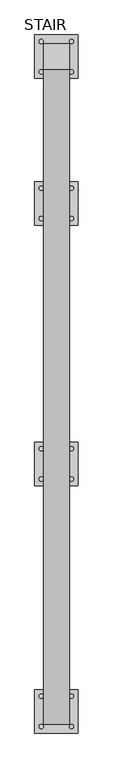
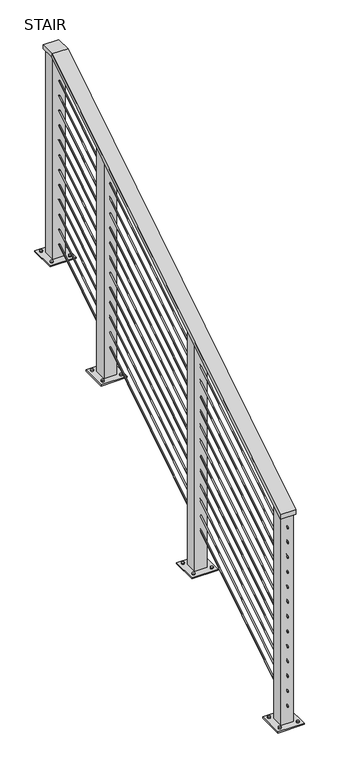
"""IFC4 building model written with IfcOpenShell, lengths in millimetres: railing geometry, STAIR."""

from ifc_helpers import new_model, si_unit, point, frame, frame_2d, origin, place, context, project, spatial, polyline, circle_curve, ellipse_curve, trimmed, segment, composite_curve, outline, extrude, faceted_brep, source, transform, mapped, element, save
from ifc_brep_helpers import plane_surface, cylinder_surface, advanced_brep


def stair_dfb8d1b2(model_context):
    return source(origin(), model_context, "Body", "SolidModel", [
        faceted_brep([(27131.1620052, 3906.3043237, 2667.5780048), (27054.9620052, 3906.3043237, 2667.5780048), (27054.9620052, 3906.3043237, 2645.0989839), (27131.1620052, 3906.3043237, 2645.0989839), (27131.1620052, 5821.2673274, 3867.15), (27054.9620052, 5821.2673274, 3867.15), (27054.9620052, 5826.7413199, 3848.1), (27131.1620052, 5826.7413199, 3848.1), (27131.1620052, 5897.4594438, 3867.15), (27131.1620052, 5897.4594438, 3848.1), (27054.9620052, 5897.4594438, 3848.1), (27054.9620052, 5897.4594438, 3867.15)], [[[0, 1, 2, 3]], [[1, 0, 4, 5]], [[2, 1, 5, 6]], [[3, 2, 6, 7]], [[0, 3, 7, 4]], [[8, 9, 10, 11]], [[5, 4, 8, 11]], [[6, 5, 11, 10]], [[7, 6, 10, 9]], [[4, 7, 9, 8]]]),
        advanced_brep(
        [(27090.6807552, 3906.3043237, 2586.8536167), (27095.4432552, 3906.3043237, 2586.8536167), (27090.6807552, 5824.6885727, 3788.56875), (27095.4432552, 5824.6885727, 3788.56875), (27090.6807552, 5897.4594438, 3788.56875), (27095.4432552, 5897.4594438, 3788.56875)],
        [
            (0, 1, ellipse_curve(frame((27093.0620052, 3906.3043237, 2586.8536167), z_axis=(0.0, -1.0, 0.0), x_axis=(0.0, 0.0, -1.0)), 2.8098776, 2.38125)),
            (1, 0, ellipse_curve(frame((27093.0620052, 3906.3043237, 2586.8536167), z_axis=(0.0, -1.0, 0.0), x_axis=(0.0, 0.0, -1.0)), 2.8098776, 2.38125)),
            (0, 2),
            (2, 3, ellipse_curve(frame((27093.0620052, 5824.6885727, 3788.56875), z_axis=(0.0, -0.9611079128273461, -0.27617309771348614), x_axis=(0.0, 0.27617309771348714, -0.9611079128273459)), 2.4776094, 2.38125)),
            (3, 1),
            (3, 2, ellipse_curve(frame((27093.0620052, 5824.6885727, 3788.56875), z_axis=(0.0, -0.9611079128273461, -0.27617309771348614), x_axis=(0.0, 0.27617309771348714, -0.9611079128273459)), 2.4776094, 2.38125)),
            (4, 5, circle_curve(frame((27093.0620052, 5897.4594438, 3788.56875), z_axis=(0.0, 1.0, 0.0), x_axis=(1.0, 0.0, 0.0)), 2.38125)),
            (5, 4, circle_curve(frame((27093.0620052, 5897.4594438, 3788.56875), z_axis=(0.0, 1.0, 0.0), x_axis=(1.0, 0.0, 0.0)), 2.38125)),
            (2, 4),
            (5, 3),
        ],
        [
            plane_surface(frame((27093.0620052, 3906.3043237, 2589.6634943), z_axis=(0.0, -1.0, 0.0), x_axis=(0.0, 0.0, 1.0))),
            cylinder_surface(frame((27093.0620052, 3907.5684443, 2587.6454877), z_axis=(0.0, -0.8474568401986745, -0.5308642990449426), x_axis=(1.0, 0.0, 0.0)), 2.38125),
            plane_surface(frame((27093.0620052, 5897.4594438, 3790.95), z_axis=(0.0, 1.0, 0.0), x_axis=(0.0, 0.0, 1.0))),
            cylinder_surface(frame((27093.0620052, 5824.0043237, 3788.56875), z_axis=(0.0, -1.0, 0.0), x_axis=(1.0, 0.0, 0.0)), 2.38125),
        ],
        [
            (0, [[1, 2]]),
            (1, [[-1, 3, 4, 5]]),
            (1, [[-2, -5, 6, -3]]),
            (2, [[7, 8]]),
            (3, [[-4, 9, -8, 10]]),
            (3, [[-6, -10, -7, -9]]),
        ],
    ),
        advanced_brep(
        [(27090.6807552, 3906.3043237, 2510.6536167), (27095.4432552, 3906.3043237, 2510.6536167), (27090.6807552, 5824.6885727, 3712.36875), (27095.4432552, 5824.6885727, 3712.36875), (27090.6807552, 5897.4594438, 3712.36875), (27095.4432552, 5897.4594438, 3712.36875)],
        [
            (0, 1, ellipse_curve(frame((27093.0620052, 3906.3043237, 2510.6536167), z_axis=(0.0, -1.0, 0.0), x_axis=(0.0, 0.0, -1.0)), 2.8098776, 2.38125)),
            (1, 0, ellipse_curve(frame((27093.0620052, 3906.3043237, 2510.6536167), z_axis=(0.0, -1.0, 0.0), x_axis=(0.0, 0.0, -1.0)), 2.8098776, 2.38125)),
            (0, 2),
            (2, 3, ellipse_curve(frame((27093.0620052, 5824.6885727, 3712.36875), z_axis=(0.0, -0.9611079128273461, -0.27617309771348614), x_axis=(0.0, 0.27617309771348714, -0.9611079128273459)), 2.4776094, 2.38125)),
            (3, 1),
            (3, 2, ellipse_curve(frame((27093.0620052, 5824.6885727, 3712.36875), z_axis=(0.0, -0.9611079128273461, -0.27617309771348614), x_axis=(0.0, 0.27617309771348714, -0.9611079128273459)), 2.4776094, 2.38125)),
            (4, 5, circle_curve(frame((27093.0620052, 5897.4594438, 3712.36875), z_axis=(0.0, 1.0, 0.0), x_axis=(1.0, 0.0, 0.0)), 2.38125)),
            (5, 4, circle_curve(frame((27093.0620052, 5897.4594438, 3712.36875), z_axis=(0.0, 1.0, 0.0), x_axis=(1.0, 0.0, 0.0)), 2.38125)),
            (2, 4),
            (5, 3),
        ],
        [
            plane_surface(frame((27093.0620052, 3906.3043237, 2513.4634943), z_axis=(0.0, -1.0, 0.0), x_axis=(0.0, 0.0, 1.0))),
            cylinder_surface(frame((27093.0620052, 3907.5684443, 2511.4454877), z_axis=(0.0, -0.8474568401986745, -0.5308642990449426), x_axis=(1.0, 0.0, 0.0)), 2.38125),
            plane_surface(frame((27093.0620052, 5897.4594438, 3714.75), z_axis=(0.0, 1.0, 0.0), x_axis=(0.0, 0.0, 1.0))),
            cylinder_surface(frame((27093.0620052, 5824.0043237, 3712.36875), z_axis=(0.0, -1.0, 0.0), x_axis=(1.0, 0.0, 0.0)), 2.38125),
        ],
        [
            (0, [[1, 2]]),
            (1, [[-1, 3, 4, 5]]),
            (1, [[-2, -5, 6, -3]]),
            (2, [[7, 8]]),
            (3, [[-4, 9, -8, 10]]),
            (3, [[-6, -10, -7, -9]]),
        ],
    ),
        advanced_brep(
        [(27090.6807552, 3906.3043237, 2434.4536167), (27095.4432552, 3906.3043237, 2434.4536167), (27090.6807552, 5824.6885727, 3636.16875), (27095.4432552, 5824.6885727, 3636.16875), (27090.6807552, 5897.4594438, 3636.16875), (27095.4432552, 5897.4594438, 3636.16875)],
        [
            (0, 1, ellipse_curve(frame((27093.0620052, 3906.3043237, 2434.4536167), z_axis=(0.0, -1.0, 0.0), x_axis=(0.0, 0.0, -1.0)), 2.8098776, 2.38125)),
            (1, 0, ellipse_curve(frame((27093.0620052, 3906.3043237, 2434.4536167), z_axis=(0.0, -1.0, 0.0), x_axis=(0.0, 0.0, -1.0)), 2.8098776, 2.38125)),
            (0, 2),
            (2, 3, ellipse_curve(frame((27093.0620052, 5824.6885727, 3636.16875), z_axis=(0.0, -0.9611079128273461, -0.27617309771348614), x_axis=(0.0, 0.27617309771348714, -0.9611079128273459)), 2.4776094, 2.38125)),
            (3, 1),
            (3, 2, ellipse_curve(frame((27093.0620052, 5824.6885727, 3636.16875), z_axis=(0.0, -0.9611079128273461, -0.27617309771348614), x_axis=(0.0, 0.27617309771348714, -0.9611079128273459)), 2.4776094, 2.38125)),
            (4, 5, circle_curve(frame((27093.0620052, 5897.4594438, 3636.16875), z_axis=(0.0, 1.0, 0.0), x_axis=(1.0, 0.0, 0.0)), 2.38125)),
            (5, 4, circle_curve(frame((27093.0620052, 5897.4594438, 3636.16875), z_axis=(0.0, 1.0, 0.0), x_axis=(1.0, 0.0, 0.0)), 2.38125)),
            (2, 4),
            (5, 3),
        ],
        [
            plane_surface(frame((27093.0620052, 3906.3043237, 2437.2634943), z_axis=(0.0, -1.0, 0.0), x_axis=(0.0, 0.0, 1.0))),
            cylinder_surface(frame((27093.0620052, 3907.5684443, 2435.2454877), z_axis=(0.0, -0.8474568401986745, -0.5308642990449426), x_axis=(1.0, 0.0, 0.0)), 2.38125),
            plane_surface(frame((27093.0620052, 5897.4594438, 3638.55), z_axis=(0.0, 1.0, 0.0), x_axis=(0.0, 0.0, 1.0))),
            cylinder_surface(frame((27093.0620052, 5824.0043237, 3636.16875), z_axis=(0.0, -1.0, 0.0), x_axis=(1.0, 0.0, 0.0)), 2.38125),
        ],
        [
            (0, [[1, 2]]),
            (1, [[-1, 3, 4, 5]]),
            (1, [[-2, -5, 6, -3]]),
            (2, [[7, 8]]),
            (3, [[-4, 9, -8, 10]]),
            (3, [[-6, -10, -7, -9]]),
        ],
    ),
        advanced_brep(
        [(27090.6807552, 3906.3043237, 2358.2536167), (27095.4432552, 3906.3043237, 2358.2536167), (27090.6807552, 5824.6885727, 3559.96875), (27095.4432552, 5824.6885727, 3559.96875), (27090.6807552, 5897.4594438, 3559.96875), (27095.4432552, 5897.4594438, 3559.96875)],
        [
            (0, 1, ellipse_curve(frame((27093.0620052, 3906.3043237, 2358.2536167), z_axis=(0.0, -1.0, 0.0), x_axis=(0.0, 0.0, -1.0)), 2.8098776, 2.38125)),
            (1, 0, ellipse_curve(frame((27093.0620052, 3906.3043237, 2358.2536167), z_axis=(0.0, -1.0, 0.0), x_axis=(0.0, 0.0, -1.0)), 2.8098776, 2.38125)),
            (0, 2),
            (2, 3, ellipse_curve(frame((27093.0620052, 5824.6885727, 3559.96875), z_axis=(0.0, -0.9611079128273461, -0.27617309771348614), x_axis=(0.0, 0.27617309771348714, -0.9611079128273459)), 2.4776094, 2.38125)),
            (3, 1),
            (3, 2, ellipse_curve(frame((27093.0620052, 5824.6885727, 3559.96875), z_axis=(0.0, -0.9611079128273461, -0.27617309771348614), x_axis=(0.0, 0.27617309771348714, -0.9611079128273459)), 2.4776094, 2.38125)),
            (4, 5, circle_curve(frame((27093.0620052, 5897.4594438, 3559.96875), z_axis=(0.0, 1.0, 0.0), x_axis=(1.0, 0.0, 0.0)), 2.38125)),
            (5, 4, circle_curve(frame((27093.0620052, 5897.4594438, 3559.96875), z_axis=(0.0, 1.0, 0.0), x_axis=(1.0, 0.0, 0.0)), 2.38125)),
            (2, 4),
            (5, 3),
        ],
        [
            plane_surface(frame((27093.0620052, 3906.3043237, 2361.0634943), z_axis=(0.0, -1.0, 0.0), x_axis=(0.0, 0.0, 1.0))),
            cylinder_surface(frame((27093.0620052, 3907.5684443, 2359.0454877), z_axis=(0.0, -0.8474568401986745, -0.5308642990449426), x_axis=(1.0, 0.0, 0.0)), 2.38125),
            plane_surface(frame((27093.0620052, 5897.4594438, 3562.35), z_axis=(0.0, 1.0, 0.0), x_axis=(0.0, 0.0, 1.0))),
            cylinder_surface(frame((27093.0620052, 5824.0043237, 3559.96875), z_axis=(0.0, -1.0, 0.0), x_axis=(1.0, 0.0, 0.0)), 2.38125),
        ],
        [
            (0, [[1, 2]]),
            (1, [[-1, 3, 4, 5]]),
            (1, [[-2, -5, 6, -3]]),
            (2, [[7, 8]]),
            (3, [[-4, 9, -8, 10]]),
            (3, [[-6, -10, -7, -9]]),
        ],
    ),
        advanced_brep(
        [(27090.6807552, 3906.3043237, 2282.0536167), (27095.4432552, 3906.3043237, 2282.0536167), (27090.6807552, 5824.6885727, 3483.76875), (27095.4432552, 5824.6885727, 3483.76875), (27090.6807552, 5897.4594438, 3483.76875), (27095.4432552, 5897.4594438, 3483.76875)],
        [
            (0, 1, ellipse_curve(frame((27093.0620052, 3906.3043237, 2282.0536167), z_axis=(0.0, -1.0, 0.0), x_axis=(0.0, 0.0, -1.0)), 2.8098776, 2.38125)),
            (1, 0, ellipse_curve(frame((27093.0620052, 3906.3043237, 2282.0536167), z_axis=(0.0, -1.0, 0.0), x_axis=(0.0, 0.0, -1.0)), 2.8098776, 2.38125)),
            (0, 2),
            (2, 3, ellipse_curve(frame((27093.0620052, 5824.6885727, 3483.76875), z_axis=(0.0, -0.9611079128273461, -0.27617309771348614), x_axis=(0.0, 0.27617309771348714, -0.9611079128273459)), 2.4776094, 2.38125)),
            (3, 1),
            (3, 2, ellipse_curve(frame((27093.0620052, 5824.6885727, 3483.76875), z_axis=(0.0, -0.9611079128273461, -0.27617309771348614), x_axis=(0.0, 0.27617309771348714, -0.9611079128273459)), 2.4776094, 2.38125)),
            (4, 5, circle_curve(frame((27093.0620052, 5897.4594438, 3483.76875), z_axis=(0.0, 1.0, 0.0), x_axis=(1.0, 0.0, 0.0)), 2.38125)),
            (5, 4, circle_curve(frame((27093.0620052, 5897.4594438, 3483.76875), z_axis=(0.0, 1.0, 0.0), x_axis=(1.0, 0.0, 0.0)), 2.38125)),
            (2, 4),
            (5, 3),
        ],
        [
            plane_surface(frame((27093.0620052, 3906.3043237, 2284.8634943), z_axis=(0.0, -1.0, 0.0), x_axis=(0.0, 0.0, 1.0))),
            cylinder_surface(frame((27093.0620052, 3907.5684443, 2282.8454877), z_axis=(0.0, -0.8474568401986745, -0.5308642990449426), x_axis=(1.0, 0.0, 0.0)), 2.38125),
            plane_surface(frame((27093.0620052, 5897.4594438, 3486.15), z_axis=(0.0, 1.0, 0.0), x_axis=(0.0, 0.0, 1.0))),
            cylinder_surface(frame((27093.0620052, 5824.0043237, 3483.76875), z_axis=(0.0, -1.0, 0.0), x_axis=(1.0, 0.0, 0.0)), 2.38125),
        ],
        [
            (0, [[1, 2]]),
            (1, [[-1, 3, 4, 5]]),
            (1, [[-2, -5, 6, -3]]),
            (2, [[7, 8]]),
            (3, [[-4, 9, -8, 10]]),
            (3, [[-6, -10, -7, -9]]),
        ],
    ),
        advanced_brep(
        [(27090.6807552, 3906.3043237, 2205.8536167), (27095.4432552, 3906.3043237, 2205.8536167), (27090.6807552, 5824.6885727, 3407.56875), (27095.4432552, 5824.6885727, 3407.56875), (27090.6807552, 5897.4594438, 3407.56875), (27095.4432552, 5897.4594438, 3407.56875)],
        [
            (0, 1, ellipse_curve(frame((27093.0620052, 3906.3043237, 2205.8536167), z_axis=(0.0, -1.0, 0.0), x_axis=(0.0, 0.0, -1.0)), 2.8098776, 2.38125)),
            (1, 0, ellipse_curve(frame((27093.0620052, 3906.3043237, 2205.8536167), z_axis=(0.0, -1.0, 0.0), x_axis=(0.0, 0.0, -1.0)), 2.8098776, 2.38125)),
            (0, 2),
            (2, 3, ellipse_curve(frame((27093.0620052, 5824.6885727, 3407.56875), z_axis=(0.0, -0.9611079128273461, -0.27617309771348614), x_axis=(0.0, 0.27617309771348714, -0.9611079128273459)), 2.4776094, 2.38125)),
            (3, 1),
            (3, 2, ellipse_curve(frame((27093.0620052, 5824.6885727, 3407.56875), z_axis=(0.0, -0.9611079128273461, -0.27617309771348614), x_axis=(0.0, 0.27617309771348714, -0.9611079128273459)), 2.4776094, 2.38125)),
            (4, 5, circle_curve(frame((27093.0620052, 5897.4594438, 3407.56875), z_axis=(0.0, 1.0, 0.0), x_axis=(1.0, 0.0, 0.0)), 2.38125)),
            (5, 4, circle_curve(frame((27093.0620052, 5897.4594438, 3407.56875), z_axis=(0.0, 1.0, 0.0), x_axis=(1.0, 0.0, 0.0)), 2.38125)),
            (2, 4),
            (5, 3),
        ],
        [
            plane_surface(frame((27093.0620052, 3906.3043237, 2208.6634943), z_axis=(0.0, -1.0, 0.0), x_axis=(0.0, 0.0, 1.0))),
            cylinder_surface(frame((27093.0620052, 3907.5684443, 2206.6454877), z_axis=(0.0, -0.8474568401986745, -0.5308642990449426), x_axis=(1.0, 0.0, 0.0)), 2.38125),
            plane_surface(frame((27093.0620052, 5897.4594438, 3409.95), z_axis=(0.0, 1.0, 0.0), x_axis=(0.0, 0.0, 1.0))),
            cylinder_surface(frame((27093.0620052, 5824.0043237, 3407.56875), z_axis=(0.0, -1.0, 0.0), x_axis=(1.0, 0.0, 0.0)), 2.38125),
        ],
        [
            (0, [[1, 2]]),
            (1, [[-1, 3, 4, 5]]),
            (1, [[-2, -5, 6, -3]]),
            (2, [[7, 8]]),
            (3, [[-4, 9, -8, 10]]),
            (3, [[-6, -10, -7, -9]]),
        ],
    ),
        advanced_brep(
        [(27090.6807552, 3906.3043237, 2129.6536167), (27095.4432552, 3906.3043237, 2129.6536167), (27090.6807552, 5824.6885727, 3331.36875), (27095.4432552, 5824.6885727, 3331.36875), (27090.6807552, 5897.4594438, 3331.36875), (27095.4432552, 5897.4594438, 3331.36875)],
        [
            (0, 1, ellipse_curve(frame((27093.0620052, 3906.3043237, 2129.6536167), z_axis=(0.0, -1.0, 0.0), x_axis=(0.0, 0.0, -1.0)), 2.8098776, 2.38125)),
            (1, 0, ellipse_curve(frame((27093.0620052, 3906.3043237, 2129.6536167), z_axis=(0.0, -1.0, 0.0), x_axis=(0.0, 0.0, -1.0)), 2.8098776, 2.38125)),
            (0, 2),
            (2, 3, ellipse_curve(frame((27093.0620052, 5824.6885727, 3331.36875), z_axis=(0.0, -0.9611079128273461, -0.27617309771348614), x_axis=(0.0, 0.27617309771348714, -0.9611079128273459)), 2.4776094, 2.38125)),
            (3, 1),
            (3, 2, ellipse_curve(frame((27093.0620052, 5824.6885727, 3331.36875), z_axis=(0.0, -0.9611079128273461, -0.27617309771348614), x_axis=(0.0, 0.27617309771348714, -0.9611079128273459)), 2.4776094, 2.38125)),
            (4, 5, circle_curve(frame((27093.0620052, 5897.4594438, 3331.36875), z_axis=(0.0, 1.0, 0.0), x_axis=(1.0, 0.0, 0.0)), 2.38125)),
            (5, 4, circle_curve(frame((27093.0620052, 5897.4594438, 3331.36875), z_axis=(0.0, 1.0, 0.0), x_axis=(1.0, 0.0, 0.0)), 2.38125)),
            (2, 4),
            (5, 3),
        ],
        [
            plane_surface(frame((27093.0620052, 3906.3043237, 2132.4634943), z_axis=(0.0, -1.0, 0.0), x_axis=(0.0, 0.0, 1.0))),
            cylinder_surface(frame((27093.0620052, 3907.5684443, 2130.4454877), z_axis=(0.0, -0.8474568401986745, -0.5308642990449426), x_axis=(1.0, 0.0, 0.0)), 2.38125),
            plane_surface(frame((27093.0620052, 5897.4594438, 3333.75), z_axis=(0.0, 1.0, 0.0), x_axis=(0.0, 0.0, 1.0))),
            cylinder_surface(frame((27093.0620052, 5824.0043237, 3331.36875), z_axis=(0.0, -1.0, 0.0), x_axis=(1.0, 0.0, 0.0)), 2.38125),
        ],
        [
            (0, [[1, 2]]),
            (1, [[-1, 3, 4, 5]]),
            (1, [[-2, -5, 6, -3]]),
            (2, [[7, 8]]),
            (3, [[-4, 9, -8, 10]]),
            (3, [[-6, -10, -7, -9]]),
        ],
    ),
        advanced_brep(
        [(27090.6807552, 3906.3043237, 2053.4536167), (27095.4432552, 3906.3043237, 2053.4536167), (27090.6807552, 5824.6885727, 3255.16875), (27095.4432552, 5824.6885727, 3255.16875), (27090.6807552, 5897.4594438, 3255.16875), (27095.4432552, 5897.4594438, 3255.16875)],
        [
            (0, 1, ellipse_curve(frame((27093.0620052, 3906.3043237, 2053.4536167), z_axis=(0.0, -1.0, 0.0), x_axis=(0.0, 0.0, -1.0)), 2.8098776, 2.38125)),
            (1, 0, ellipse_curve(frame((27093.0620052, 3906.3043237, 2053.4536167), z_axis=(0.0, -1.0, 0.0), x_axis=(0.0, 0.0, -1.0)), 2.8098776, 2.38125)),
            (0, 2),
            (2, 3, ellipse_curve(frame((27093.0620052, 5824.6885727, 3255.16875), z_axis=(0.0, -0.9611079128273461, -0.27617309771348614), x_axis=(0.0, 0.27617309771348714, -0.9611079128273459)), 2.4776094, 2.38125)),
            (3, 1),
            (3, 2, ellipse_curve(frame((27093.0620052, 5824.6885727, 3255.16875), z_axis=(0.0, -0.9611079128273461, -0.27617309771348614), x_axis=(0.0, 0.27617309771348714, -0.9611079128273459)), 2.4776094, 2.38125)),
            (4, 5, circle_curve(frame((27093.0620052, 5897.4594438, 3255.16875), z_axis=(0.0, 1.0, 0.0), x_axis=(1.0, 0.0, 0.0)), 2.38125)),
            (5, 4, circle_curve(frame((27093.0620052, 5897.4594438, 3255.16875), z_axis=(0.0, 1.0, 0.0), x_axis=(1.0, 0.0, 0.0)), 2.38125)),
            (2, 4),
            (5, 3),
        ],
        [
            plane_surface(frame((27093.0620052, 3906.3043237, 2056.2634943), z_axis=(0.0, -1.0, 0.0), x_axis=(0.0, 0.0, 1.0))),
            cylinder_surface(frame((27093.0620052, 3907.5684443, 2054.2454877), z_axis=(0.0, -0.8474568401986745, -0.5308642990449426), x_axis=(1.0, 0.0, 0.0)), 2.38125),
            plane_surface(frame((27093.0620052, 5897.4594438, 3257.55), z_axis=(0.0, 1.0, 0.0), x_axis=(0.0, 0.0, 1.0))),
            cylinder_surface(frame((27093.0620052, 5824.0043237, 3255.16875), z_axis=(0.0, -1.0, 0.0), x_axis=(1.0, 0.0, 0.0)), 2.38125),
        ],
        [
            (0, [[1, 2]]),
            (1, [[-1, 3, 4, 5]]),
            (1, [[-2, -5, 6, -3]]),
            (2, [[7, 8]]),
            (3, [[-4, 9, -8, 10]]),
            (3, [[-6, -10, -7, -9]]),
        ],
    ),
        advanced_brep(
        [(27090.6807552, 3906.3043237, 1977.2536167), (27095.4432552, 3906.3043237, 1977.2536167), (27090.6807552, 5824.6885727, 3178.96875), (27095.4432552, 5824.6885727, 3178.96875), (27090.6807552, 5897.4594438, 3178.96875), (27095.4432552, 5897.4594438, 3178.96875)],
        [
            (0, 1, ellipse_curve(frame((27093.0620052, 3906.3043237, 1977.2536167), z_axis=(0.0, -1.0, 0.0), x_axis=(0.0, 0.0, -1.0)), 2.8098776, 2.38125)),
            (1, 0, ellipse_curve(frame((27093.0620052, 3906.3043237, 1977.2536167), z_axis=(0.0, -1.0, 0.0), x_axis=(0.0, 0.0, -1.0)), 2.8098776, 2.38125)),
            (0, 2),
            (2, 3, ellipse_curve(frame((27093.0620052, 5824.6885727, 3178.96875), z_axis=(0.0, -0.9611079128273461, -0.27617309771348614), x_axis=(0.0, 0.27617309771348714, -0.9611079128273459)), 2.4776094, 2.38125)),
            (3, 1),
            (3, 2, ellipse_curve(frame((27093.0620052, 5824.6885727, 3178.96875), z_axis=(0.0, -0.9611079128273461, -0.27617309771348614), x_axis=(0.0, 0.27617309771348714, -0.9611079128273459)), 2.4776094, 2.38125)),
            (4, 5, circle_curve(frame((27093.0620052, 5897.4594438, 3178.96875), z_axis=(0.0, 1.0, 0.0), x_axis=(1.0, 0.0, 0.0)), 2.38125)),
            (5, 4, circle_curve(frame((27093.0620052, 5897.4594438, 3178.96875), z_axis=(0.0, 1.0, 0.0), x_axis=(1.0, 0.0, 0.0)), 2.38125)),
            (2, 4),
            (5, 3),
        ],
        [
            plane_surface(frame((27093.0620052, 3906.3043237, 1980.0634943), z_axis=(0.0, -1.0, 0.0), x_axis=(0.0, 0.0, 1.0))),
            cylinder_surface(frame((27093.0620052, 3907.5684443, 1978.0454877), z_axis=(0.0, -0.8474568401986745, -0.5308642990449426), x_axis=(1.0, 0.0, 0.0)), 2.38125),
            plane_surface(frame((27093.0620052, 5897.4594438, 3181.35), z_axis=(0.0, 1.0, 0.0), x_axis=(0.0, 0.0, 1.0))),
            cylinder_surface(frame((27093.0620052, 5824.0043237, 3178.96875), z_axis=(0.0, -1.0, 0.0), x_axis=(1.0, 0.0, 0.0)), 2.38125),
        ],
        [
            (0, [[1, 2]]),
            (1, [[-1, 3, 4, 5]]),
            (1, [[-2, -5, 6, -3]]),
            (2, [[7, 8]]),
            (3, [[-4, 9, -8, 10]]),
            (3, [[-6, -10, -7, -9]]),
        ],
    ),
        advanced_brep(
        [(27090.6807552, 3906.3043237, 1901.0536167), (27095.4432552, 3906.3043237, 1901.0536167), (27090.6807552, 5824.6885727, 3102.76875), (27095.4432552, 5824.6885727, 3102.76875), (27090.6807552, 5897.4594438, 3102.76875), (27095.4432552, 5897.4594438, 3102.76875)],
        [
            (0, 1, ellipse_curve(frame((27093.0620052, 3906.3043237, 1901.0536167), z_axis=(0.0, -1.0, 0.0), x_axis=(0.0, 0.0, -1.0)), 2.8098776, 2.38125)),
            (1, 0, ellipse_curve(frame((27093.0620052, 3906.3043237, 1901.0536167), z_axis=(0.0, -1.0, 0.0), x_axis=(0.0, 0.0, -1.0)), 2.8098776, 2.38125)),
            (0, 2),
            (2, 3, ellipse_curve(frame((27093.0620052, 5824.6885727, 3102.76875), z_axis=(0.0, -0.9611079128273461, -0.27617309771348614), x_axis=(0.0, 0.27617309771348714, -0.9611079128273459)), 2.4776094, 2.38125)),
            (3, 1),
            (3, 2, ellipse_curve(frame((27093.0620052, 5824.6885727, 3102.76875), z_axis=(0.0, -0.9611079128273461, -0.27617309771348614), x_axis=(0.0, 0.27617309771348714, -0.9611079128273459)), 2.4776094, 2.38125)),
            (4, 5, circle_curve(frame((27093.0620052, 5897.4594438, 3102.76875), z_axis=(0.0, 1.0, 0.0), x_axis=(1.0, 0.0, 0.0)), 2.38125)),
            (5, 4, circle_curve(frame((27093.0620052, 5897.4594438, 3102.76875), z_axis=(0.0, 1.0, 0.0), x_axis=(1.0, 0.0, 0.0)), 2.38125)),
            (2, 4),
            (5, 3),
        ],
        [
            plane_surface(frame((27093.0620052, 3906.3043237, 1903.8634943), z_axis=(0.0, -1.0, 0.0), x_axis=(0.0, 0.0, 1.0))),
            cylinder_surface(frame((27093.0620052, 3907.5684443, 1901.8454877), z_axis=(0.0, -0.8474568401986745, -0.5308642990449426), x_axis=(1.0, 0.0, 0.0)), 2.38125),
            plane_surface(frame((27093.0620052, 5897.4594438, 3105.15), z_axis=(0.0, 1.0, 0.0), x_axis=(0.0, 0.0, 1.0))),
            cylinder_surface(frame((27093.0620052, 5824.0043237, 3102.76875), z_axis=(0.0, -1.0, 0.0), x_axis=(1.0, 0.0, 0.0)), 2.38125),
        ],
        [
            (0, [[1, 2]]),
            (1, [[-1, 3, 4, 5]]),
            (1, [[-2, -5, 6, -3]]),
            (2, [[7, 8]]),
            (3, [[-4, 9, -8, 10]]),
            (3, [[-6, -10, -7, -9]]),
        ],
    ),
        advanced_brep(
        [(27090.6807552, 3906.3043237, 1824.8536167), (27095.4432552, 3906.3043237, 1824.8536167), (27090.6807552, 5824.6885727, 3026.56875), (27095.4432552, 5824.6885727, 3026.56875), (27090.6807552, 5897.4594438, 3026.56875), (27095.4432552, 5897.4594438, 3026.56875)],
        [
            (0, 1, ellipse_curve(frame((27093.0620052, 3906.3043237, 1824.8536167), z_axis=(0.0, -1.0, 0.0), x_axis=(0.0, 0.0, -1.0)), 2.8098776, 2.38125)),
            (1, 0, ellipse_curve(frame((27093.0620052, 3906.3043237, 1824.8536167), z_axis=(0.0, -1.0, 0.0), x_axis=(0.0, 0.0, -1.0)), 2.8098776, 2.38125)),
            (0, 2),
            (2, 3, ellipse_curve(frame((27093.0620052, 5824.6885727, 3026.56875), z_axis=(0.0, -0.9611079128273461, -0.27617309771348614), x_axis=(0.0, 0.27617309771348714, -0.9611079128273459)), 2.4776094, 2.38125)),
            (3, 1),
            (3, 2, ellipse_curve(frame((27093.0620052, 5824.6885727, 3026.56875), z_axis=(0.0, -0.9611079128273461, -0.27617309771348614), x_axis=(0.0, 0.27617309771348714, -0.9611079128273459)), 2.4776094, 2.38125)),
            (4, 5, circle_curve(frame((27093.0620052, 5897.4594438, 3026.56875), z_axis=(0.0, 1.0, 0.0), x_axis=(1.0, 0.0, 0.0)), 2.38125)),
            (5, 4, circle_curve(frame((27093.0620052, 5897.4594438, 3026.56875), z_axis=(0.0, 1.0, 0.0), x_axis=(1.0, 0.0, 0.0)), 2.38125)),
            (2, 4),
            (5, 3),
        ],
        [
            plane_surface(frame((27093.0620052, 3906.3043237, 1827.6634943), z_axis=(0.0, -1.0, 0.0), x_axis=(0.0, 0.0, 1.0))),
            cylinder_surface(frame((27093.0620052, 3907.5684443, 1825.6454877), z_axis=(0.0, -0.8474568401986745, -0.5308642990449426), x_axis=(1.0, 0.0, 0.0)), 2.38125),
            plane_surface(frame((27093.0620052, 5897.4594438, 3028.95), z_axis=(0.0, 1.0, 0.0), x_axis=(0.0, 0.0, 1.0))),
            cylinder_surface(frame((27093.0620052, 5824.0043237, 3026.56875), z_axis=(0.0, -1.0, 0.0), x_axis=(1.0, 0.0, 0.0)), 2.38125),
        ],
        [
            (0, [[1, 2]]),
            (1, [[-1, 3, 4, 5]]),
            (1, [[-2, -5, 6, -3]]),
            (2, [[7, 8]]),
            (3, [[-4, 9, -8, 10]]),
            (3, [[-6, -10, -7, -9]]),
        ],
    ),
        advanced_brep(
        [(27090.6807552, 3906.3043237, 1748.6536167), (27095.4432552, 3906.3043237, 1748.6536167), (27090.6807552, 5824.6885727, 2950.36875), (27095.4432552, 5824.6885727, 2950.36875), (27090.6807552, 5897.4594438, 2950.36875), (27095.4432552, 5897.4594438, 2950.36875)],
        [
            (0, 1, ellipse_curve(frame((27093.0620052, 3906.3043237, 1748.6536167), z_axis=(0.0, -1.0, 0.0), x_axis=(0.0, 0.0, -1.0)), 2.8098776, 2.38125)),
            (1, 0, ellipse_curve(frame((27093.0620052, 3906.3043237, 1748.6536167), z_axis=(0.0, -1.0, 0.0), x_axis=(0.0, 0.0, -1.0)), 2.8098776, 2.38125)),
            (0, 2),
            (2, 3, ellipse_curve(frame((27093.0620052, 5824.6885727, 2950.36875), z_axis=(0.0, -0.9611079128273461, -0.27617309771348614), x_axis=(0.0, 0.27617309771348714, -0.9611079128273459)), 2.4776094, 2.38125)),
            (3, 1),
            (3, 2, ellipse_curve(frame((27093.0620052, 5824.6885727, 2950.36875), z_axis=(0.0, -0.9611079128273461, -0.27617309771348614), x_axis=(0.0, 0.27617309771348714, -0.9611079128273459)), 2.4776094, 2.38125)),
            (4, 5, circle_curve(frame((27093.0620052, 5897.4594438, 2950.36875), z_axis=(0.0, 1.0, 0.0), x_axis=(1.0, 0.0, 0.0)), 2.38125)),
            (5, 4, circle_curve(frame((27093.0620052, 5897.4594438, 2950.36875), z_axis=(0.0, 1.0, 0.0), x_axis=(1.0, 0.0, 0.0)), 2.38125)),
            (2, 4),
            (5, 3),
        ],
        [
            plane_surface(frame((27093.0620052, 3906.3043237, 1751.4634943), z_axis=(0.0, -1.0, 0.0), x_axis=(0.0, 0.0, 1.0))),
            cylinder_surface(frame((27093.0620052, 3907.5684443, 1749.4454877), z_axis=(0.0, -0.8474568401986745, -0.5308642990449426), x_axis=(1.0, 0.0, 0.0)), 2.38125),
            plane_surface(frame((27093.0620052, 5897.4594438, 2952.75), z_axis=(0.0, 1.0, 0.0), x_axis=(0.0, 0.0, 1.0))),
            cylinder_surface(frame((27093.0620052, 5824.0043237, 2950.36875), z_axis=(0.0, -1.0, 0.0), x_axis=(1.0, 0.0, 0.0)), 2.38125),
        ],
        [
            (0, [[1, 2]]),
            (1, [[-1, 3, 4, 5]]),
            (1, [[-2, -5, 6, -3]]),
            (2, [[7, 8]]),
            (3, [[-4, 9, -8, 10]]),
            (3, [[-6, -10, -7, -9]]),
        ],
    ),
        advanced_brep(
        [(27090.6807552, 3906.3043237, 1672.4536167), (27095.4432552, 3906.3043237, 1672.4536167), (27090.6807552, 5824.6885727, 2874.16875), (27095.4432552, 5824.6885727, 2874.16875), (27090.6807552, 5897.4594438, 2874.16875), (27095.4432552, 5897.4594438, 2874.16875)],
        [
            (0, 1, ellipse_curve(frame((27093.0620052, 3906.3043237, 1672.4536167), z_axis=(0.0, -1.0, 0.0), x_axis=(0.0, 0.0, -1.0)), 2.8098776, 2.38125)),
            (1, 0, ellipse_curve(frame((27093.0620052, 3906.3043237, 1672.4536167), z_axis=(0.0, -1.0, 0.0), x_axis=(0.0, 0.0, -1.0)), 2.8098776, 2.38125)),
            (0, 2),
            (2, 3, ellipse_curve(frame((27093.0620052, 5824.6885727, 2874.16875), z_axis=(0.0, -0.9611079128273461, -0.27617309771348614), x_axis=(0.0, 0.27617309771348714, -0.9611079128273459)), 2.4776094, 2.38125)),
            (3, 1),
            (3, 2, ellipse_curve(frame((27093.0620052, 5824.6885727, 2874.16875), z_axis=(0.0, -0.9611079128273461, -0.27617309771348614), x_axis=(0.0, 0.27617309771348714, -0.9611079128273459)), 2.4776094, 2.38125)),
            (4, 5, circle_curve(frame((27093.0620052, 5897.4594438, 2874.16875), z_axis=(0.0, 1.0, 0.0), x_axis=(1.0, 0.0, 0.0)), 2.38125)),
            (5, 4, circle_curve(frame((27093.0620052, 5897.4594438, 2874.16875), z_axis=(0.0, 1.0, 0.0), x_axis=(1.0, 0.0, 0.0)), 2.38125)),
            (2, 4),
            (5, 3),
        ],
        [
            plane_surface(frame((27093.0620052, 3906.3043237, 1675.2634943), z_axis=(0.0, -1.0, 0.0), x_axis=(0.0, 0.0, 1.0))),
            cylinder_surface(frame((27093.0620052, 3907.5684443, 1673.2454877), z_axis=(0.0, -0.8474568401986745, -0.5308642990449426), x_axis=(1.0, 0.0, 0.0)), 2.38125),
            plane_surface(frame((27093.0620052, 5897.4594438, 2876.55), z_axis=(0.0, 1.0, 0.0), x_axis=(0.0, 0.0, 1.0))),
            cylinder_surface(frame((27093.0620052, 5824.0043237, 2874.16875), z_axis=(0.0, -1.0, 0.0), x_axis=(1.0, 0.0, 0.0)), 2.38125),
        ],
        [
            (0, [[1, 2]]),
            (1, [[-1, 3, 4, 5]]),
            (1, [[-2, -5, 6, -3]]),
            (2, [[7, 8]]),
            (3, [[-4, 9, -8, 10]]),
            (3, [[-6, -10, -7, -9]]),
        ],
    ),
        extrude(outline(composite_curve([segment(trimmed(circle_curve(frame_2d((27137.5120052, 5385.8543237)), 6.35), [point((27143.8620052, 5385.8543237))], [point((27131.1620052, 5385.8543237))], False, "CARTESIAN"), True, "CONTINUOUS"), segment(trimmed(circle_curve(frame_2d((27137.5120052, 5385.8543237)), 6.35), [point((27131.1620052, 5385.8543237))], [point((27143.8620052, 5385.8543237))], False, "CARTESIAN"), True, "CONTINUOUS")], self_intersect=False)), frame((0.0, 0.0, 2450.30625), z_axis=(0.0, 0.0, 1.0), x_axis=(1.0, 0.0, 0.0)), (0.0, 0.0, 1.0), 12.7),
        extrude(outline(composite_curve([segment(trimmed(circle_curve(frame_2d((27048.6120052, 5385.8543237)), 6.35), [point((27054.9620052, 5385.8543237))], [point((27042.2620052, 5385.8543237))], False, "CARTESIAN"), True, "CONTINUOUS"), segment(trimmed(circle_curve(frame_2d((27048.6120052, 5385.8543237)), 6.35), [point((27042.2620052, 5385.8543237))], [point((27054.9620052, 5385.8543237))], False, "CARTESIAN"), True, "CONTINUOUS")], self_intersect=False)), frame((0.0, 0.0, 2450.30625), z_axis=(0.0, 0.0, 1.0), x_axis=(1.0, 0.0, 0.0)), (0.0, 0.0, 1.0), 12.7),
        extrude(outline(composite_curve([segment(trimmed(circle_curve(frame_2d((27137.5120052, 5474.7543237)), 6.35), [point((27143.8620052, 5474.7543237))], [point((27131.1620052, 5474.7543237))], False, "CARTESIAN"), True, "CONTINUOUS"), segment(trimmed(circle_curve(frame_2d((27137.5120052, 5474.7543237)), 6.35), [point((27131.1620052, 5474.7543237))], [point((27143.8620052, 5474.7543237))], False, "CARTESIAN"), True, "CONTINUOUS")], self_intersect=False)), frame((0.0, 0.0, 2450.30625), z_axis=(0.0, 0.0, 1.0), x_axis=(1.0, 0.0, 0.0)), (0.0, 0.0, 1.0), 12.7),
        extrude(outline(composite_curve([segment(trimmed(circle_curve(frame_2d((27048.6120052, 5474.7543237)), 6.35), [point((27054.9620052, 5474.7543237))], [point((27042.2620052, 5474.7543237))], False, "CARTESIAN"), True, "CONTINUOUS"), segment(trimmed(circle_curve(frame_2d((27048.6120052, 5474.7543237)), 6.35), [point((27042.2620052, 5474.7543237))], [point((27054.9620052, 5474.7543237))], False, "CARTESIAN"), True, "CONTINUOUS")], self_intersect=False)), frame((0.0, 0.0, 2450.30625), z_axis=(0.0, 0.0, 1.0), x_axis=(1.0, 0.0, 0.0)), (0.0, 0.0, 1.0), 12.7),
        extrude(outline(polyline([(27029.5620052, 5366.8043237), (27029.5620052, 5493.8043237), (27156.5620052, 5493.8043237), (27156.5620052, 5366.8043237), (27029.5620052, 5366.8043237)])), frame((0.0, 0.0, 2450.30625), z_axis=(0.0, 0.0, 1.0), x_axis=(1.0, 0.0, 0.0)), (0.0, 0.0, 1.0), 6.35),
        extrude(outline(polyline([(27062.8995052, 5400.1418237), (27062.8995052, 5460.4668237), (27123.2245052, 5460.4668237), (27123.2245052, 5400.1418237), (27062.8995052, 5400.1418237)]), holes=[polyline([(27069.2495052, 5406.4918237), (27116.8745052, 5406.4918237), (27116.8745052, 5454.1168237), (27069.2495052, 5454.1168237), (27069.2495052, 5406.4918237)])]), frame((0.0, 0.0, 2450.30625), z_axis=(0.0, 0.0, 1.0), x_axis=(1.0, 0.0, 0.0)), (0.0, 0.0, 1.0), 1151.172017),
        extrude(outline(composite_curve([segment(trimmed(circle_curve(frame_2d((27137.5120052, 4623.8543237)), 6.35), [point((27143.8620052, 4623.8543237))], [point((27131.1620052, 4623.8543237))], False, "CARTESIAN"), True, "CONTINUOUS"), segment(trimmed(circle_curve(frame_2d((27137.5120052, 4623.8543237)), 6.35), [point((27131.1620052, 4623.8543237))], [point((27143.8620052, 4623.8543237))], False, "CARTESIAN"), True, "CONTINUOUS")], self_intersect=False)), frame((0.0, 0.0, 1925.240625), z_axis=(0.0, 0.0, 1.0), x_axis=(1.0, 0.0, 0.0)), (0.0, 0.0, 1.0), 12.7),
        extrude(outline(composite_curve([segment(trimmed(circle_curve(frame_2d((27048.6120052, 4623.8543237)), 6.35), [point((27054.9620052, 4623.8543237))], [point((27042.2620052, 4623.8543237))], False, "CARTESIAN"), True, "CONTINUOUS"), segment(trimmed(circle_curve(frame_2d((27048.6120052, 4623.8543237)), 6.35), [point((27042.2620052, 4623.8543237))], [point((27054.9620052, 4623.8543237))], False, "CARTESIAN"), True, "CONTINUOUS")], self_intersect=False)), frame((0.0, 0.0, 1925.240625), z_axis=(0.0, 0.0, 1.0), x_axis=(1.0, 0.0, 0.0)), (0.0, 0.0, 1.0), 12.7),
        extrude(outline(composite_curve([segment(trimmed(circle_curve(frame_2d((27137.5120052, 4712.7543237)), 6.35), [point((27143.8620052, 4712.7543237))], [point((27131.1620052, 4712.7543237))], False, "CARTESIAN"), True, "CONTINUOUS"), segment(trimmed(circle_curve(frame_2d((27137.5120052, 4712.7543237)), 6.35), [point((27131.1620052, 4712.7543237))], [point((27143.8620052, 4712.7543237))], False, "CARTESIAN"), True, "CONTINUOUS")], self_intersect=False)), frame((0.0, 0.0, 1925.240625), z_axis=(0.0, 0.0, 1.0), x_axis=(1.0, 0.0, 0.0)), (0.0, 0.0, 1.0), 12.7),
        extrude(outline(composite_curve([segment(trimmed(circle_curve(frame_2d((27048.6120052, 4712.7543237)), 6.35), [point((27054.9620052, 4712.7543237))], [point((27042.2620052, 4712.7543237))], False, "CARTESIAN"), True, "CONTINUOUS"), segment(trimmed(circle_curve(frame_2d((27048.6120052, 4712.7543237)), 6.35), [point((27042.2620052, 4712.7543237))], [point((27054.9620052, 4712.7543237))], False, "CARTESIAN"), True, "CONTINUOUS")], self_intersect=False)), frame((0.0, 0.0, 1925.240625), z_axis=(0.0, 0.0, 1.0), x_axis=(1.0, 0.0, 0.0)), (0.0, 0.0, 1.0), 12.7),
        extrude(outline(polyline([(27029.5620052, 4604.8043237), (27029.5620052, 4731.8043237), (27156.5620052, 4731.8043237), (27156.5620052, 4604.8043237), (27029.5620052, 4604.8043237)])), frame((0.0, 0.0, 1925.240625), z_axis=(0.0, 0.0, 1.0), x_axis=(1.0, 0.0, 0.0)), (0.0, 0.0, 1.0), 6.35),
        extrude(outline(polyline([(27062.8995052, 4638.1418237), (27062.8995052, 4698.4668237), (27123.2245052, 4698.4668237), (27123.2245052, 4638.1418237), (27062.8995052, 4638.1418237)]), holes=[polyline([(27069.2495052, 4644.4918237), (27116.8745052, 4644.4918237), (27116.8745052, 4692.1168237), (27069.2495052, 4692.1168237), (27069.2495052, 4644.4918237)])]), frame((0.0, 0.0, 1925.240625), z_axis=(0.0, 0.0, 1.0), x_axis=(1.0, 0.0, 0.0)), (0.0, 0.0, 1.0), 1198.9052557),
        extrude(outline(composite_curve([segment(trimmed(circle_curve(frame_2d((27137.5120052, 5814.9094438)), 6.35), [point((27143.8620052, 5814.9094438))], [point((27131.1620052, 5814.9094438))], False, "CARTESIAN"), True, "CONTINUOUS"), segment(trimmed(circle_curve(frame_2d((27137.5120052, 5814.9094438)), 6.35), [point((27131.1620052, 5814.9094438))], [point((27143.8620052, 5814.9094438))], False, "CARTESIAN"), True, "CONTINUOUS")], self_intersect=False)), frame((0.0, 0.0, 2800.35), z_axis=(0.0, 0.0, 1.0), x_axis=(1.0, 0.0, 0.0)), (0.0, 0.0, 1.0), 12.7),
        extrude(outline(composite_curve([segment(trimmed(circle_curve(frame_2d((27048.6120052, 5814.9094438)), 6.35), [point((27054.9620052, 5814.9094438))], [point((27042.2620052, 5814.9094438))], False, "CARTESIAN"), True, "CONTINUOUS"), segment(trimmed(circle_curve(frame_2d((27048.6120052, 5814.9094438)), 6.35), [point((27042.2620052, 5814.9094438))], [point((27054.9620052, 5814.9094438))], False, "CARTESIAN"), True, "CONTINUOUS")], self_intersect=False)), frame((0.0, 0.0, 2800.35), z_axis=(0.0, 0.0, 1.0), x_axis=(1.0, 0.0, 0.0)), (0.0, 0.0, 1.0), 12.7),
        extrude(outline(composite_curve([segment(trimmed(circle_curve(frame_2d((27137.5120052, 5903.8094438)), 6.35), [point((27143.8620052, 5903.8094438))], [point((27131.1620052, 5903.8094438))], False, "CARTESIAN"), True, "CONTINUOUS"), segment(trimmed(circle_curve(frame_2d((27137.5120052, 5903.8094438)), 6.35), [point((27131.1620052, 5903.8094438))], [point((27143.8620052, 5903.8094438))], False, "CARTESIAN"), True, "CONTINUOUS")], self_intersect=False)), frame((0.0, 0.0, 2800.35), z_axis=(0.0, 0.0, 1.0), x_axis=(1.0, 0.0, 0.0)), (0.0, 0.0, 1.0), 12.7),
        extrude(outline(composite_curve([segment(trimmed(circle_curve(frame_2d((27048.6120052, 5903.8094438)), 6.35), [point((27054.9620052, 5903.8094438))], [point((27042.2620052, 5903.8094438))], False, "CARTESIAN"), True, "CONTINUOUS"), segment(trimmed(circle_curve(frame_2d((27048.6120052, 5903.8094438)), 6.35), [point((27042.2620052, 5903.8094438))], [point((27054.9620052, 5903.8094438))], False, "CARTESIAN"), True, "CONTINUOUS")], self_intersect=False)), frame((0.0, 0.0, 2800.35), z_axis=(0.0, 0.0, 1.0), x_axis=(1.0, 0.0, 0.0)), (0.0, 0.0, 1.0), 12.7),
        extrude(outline(polyline([(27029.5620052, 5795.8594438), (27029.5620052, 5922.8594438), (27156.5620052, 5922.8594438), (27156.5620052, 5795.8594438), (27029.5620052, 5795.8594438)])), frame((0.0, 0.0, 2800.35), z_axis=(0.0, 0.0, 1.0), x_axis=(1.0, 0.0, 0.0)), (0.0, 0.0, 1.0), 6.35),
        extrude(outline(polyline([(27062.8995052, 5829.1969438), (27062.8995052, 5889.5219438), (27123.2245052, 5889.5219438), (27123.2245052, 5829.1969438), (27062.8995052, 5829.1969438)]), holes=[polyline([(27069.2495052, 5835.5469438), (27116.8745052, 5835.5469438), (27116.8745052, 5883.1719438), (27069.2495052, 5883.1719438), (27069.2495052, 5835.5469438)])]), frame((0.0, 0.0, 2800.35), z_axis=(0.0, 0.0, 1.0), x_axis=(1.0, 0.0, 0.0)), (0.0, 0.0, 1.0), 1047.75),
        extrude(outline(composite_curve([segment(trimmed(circle_curve(frame_2d((27137.5120052, 3899.9543237)), 6.35), [point((27143.8620052, 3899.9543237))], [point((27131.1620052, 3899.9543237))], False, "CARTESIAN"), True, "CONTINUOUS"), segment(trimmed(circle_curve(frame_2d((27137.5120052, 3899.9543237)), 6.35), [point((27131.1620052, 3899.9543237))], [point((27143.8620052, 3899.9543237))], False, "CARTESIAN"), True, "CONTINUOUS")], self_intersect=False)), frame((0.0, 0.0, 1575.196875), z_axis=(0.0, 0.0, 1.0), x_axis=(1.0, 0.0, 0.0)), (0.0, 0.0, 1.0), 12.7),
        extrude(outline(composite_curve([segment(trimmed(circle_curve(frame_2d((27048.6120052, 3899.9543237)), 6.35), [point((27054.9620052, 3899.9543237))], [point((27042.2620052, 3899.9543237))], False, "CARTESIAN"), True, "CONTINUOUS"), segment(trimmed(circle_curve(frame_2d((27048.6120052, 3899.9543237)), 6.35), [point((27042.2620052, 3899.9543237))], [point((27054.9620052, 3899.9543237))], False, "CARTESIAN"), True, "CONTINUOUS")], self_intersect=False)), frame((0.0, 0.0, 1575.196875), z_axis=(0.0, 0.0, 1.0), x_axis=(1.0, 0.0, 0.0)), (0.0, 0.0, 1.0), 12.7),
        extrude(outline(composite_curve([segment(trimmed(circle_curve(frame_2d((27137.5120052, 3988.8543237)), 6.35), [point((27143.8620052, 3988.8543237))], [point((27131.1620052, 3988.8543237))], False, "CARTESIAN"), True, "CONTINUOUS"), segment(trimmed(circle_curve(frame_2d((27137.5120052, 3988.8543237)), 6.35), [point((27131.1620052, 3988.8543237))], [point((27143.8620052, 3988.8543237))], False, "CARTESIAN"), True, "CONTINUOUS")], self_intersect=False)), frame((0.0, 0.0, 1575.196875), z_axis=(0.0, 0.0, 1.0), x_axis=(1.0, 0.0, 0.0)), (0.0, 0.0, 1.0), 12.7),
        extrude(outline(composite_curve([segment(trimmed(circle_curve(frame_2d((27048.6120052, 3988.8543237)), 6.35), [point((27054.9620052, 3988.8543237))], [point((27042.2620052, 3988.8543237))], False, "CARTESIAN"), True, "CONTINUOUS"), segment(trimmed(circle_curve(frame_2d((27048.6120052, 3988.8543237)), 6.35), [point((27042.2620052, 3988.8543237))], [point((27054.9620052, 3988.8543237))], False, "CARTESIAN"), True, "CONTINUOUS")], self_intersect=False)), frame((0.0, 0.0, 1575.196875), z_axis=(0.0, 0.0, 1.0), x_axis=(1.0, 0.0, 0.0)), (0.0, 0.0, 1.0), 12.7),
        extrude(outline(polyline([(27029.5620052, 3880.9043237), (27029.5620052, 4007.9043237), (27156.5620052, 4007.9043237), (27156.5620052, 3880.9043237), (27029.5620052, 3880.9043237)])), frame((0.0, 0.0, 1575.196875), z_axis=(0.0, 0.0, 1.0), x_axis=(1.0, 0.0, 0.0)), (0.0, 0.0, 1.0), 6.35),
        extrude(outline(polyline([(27062.8995052, 3914.2418237), (27062.8995052, 3974.5668237), (27123.2245052, 3974.5668237), (27123.2245052, 3914.2418237), (27062.8995052, 3914.2418237)]), holes=[polyline([(27069.2495052, 3920.5918237), (27116.8745052, 3920.5918237), (27116.8745052, 3968.2168237), (27069.2495052, 3968.2168237), (27069.2495052, 3920.5918237)])]), frame((0.0, 0.0, 1575.196875), z_axis=(0.0, 0.0, 1.0), x_axis=(1.0, 0.0, 0.0)), (0.0, 0.0, 1.0), 1095.4832386),
    ])


if __name__ == "__main__":
    model = new_model("IFC4")
    model_context = context("Model", 3, world=origin())
    ifc_project = project(units=[si_unit("LENGTHUNIT", "METRE", prefix="MILLI")], contexts=[model_context])
    site = spatial("IfcSite", under=ifc_project)
    building = spatial("IfcBuilding", under=site)
    placement = place(None, origin())
    stair_shape = stair_dfb8d1b2(model_context)
    element("IfcRailing", 1, ObjectType="STAIR", at=placement, inside=building, context=model_context, shape_type="MappedRepresentation", body=[
        mapped(stair_shape, transform((0.0, 0.0, 0.0), x_axis=(1.0, 0.0, 0.0), y_axis=(0.0, 1.0, 0.0), z_axis=(0.0, 0.0, 1.0))),
    ])
    save(model, "model.ifc")

# Revit data of these elements
# Element 1 (IfcRailing, "STAIR")
#   Materials on its faces: "2 1/2\" X 2 1/2\" ALUM. SQUARE POST (38\" O.C. MAX)", "WIRE RAILING (3\" O.C.)", "ALUM. PLATE TOP RAIL"
# Materials
#   "2 1/2\" X 2 1/2\" ALUM. SQUARE POST (38\" O.C. MAX)": class "Metal", colour RGB 244 244 244, transparency 0, Manufacturer = "Kawneer", URL = "http://www.kawneer.com/kawneer/north_america/en/home.asp", Cost = 0
#   "WIRE RAILING (3\" O.C.)": class "Metal", colour RGB 244 244 244, transparency 0, Manufacturer = "Kawneer", URL = "http://www.kawneer.com/kawneer/north_america/en/home.asp", Cost = 0
#   "ALUM. PLATE TOP RAIL": class "Metal", colour RGB 244 244 244, transparency 0, Manufacturer = "Kawneer", URL = "http://www.kawneer.com/kawneer/north_america/en/home.asp", Cost = 0
